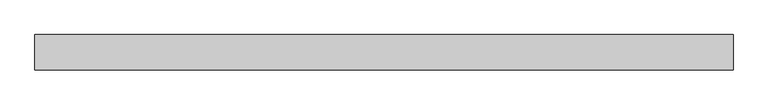
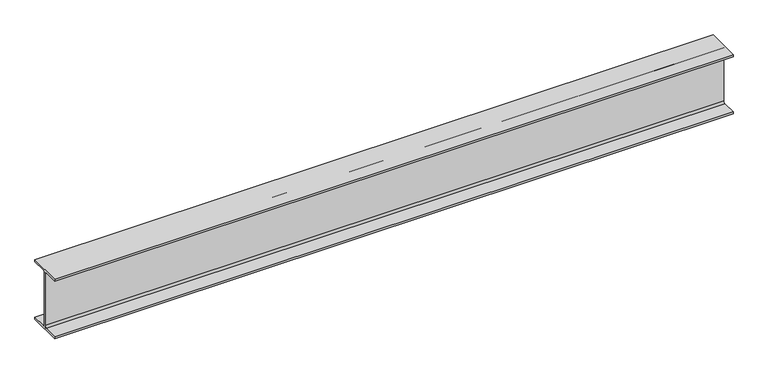
"""IFC4 building model written with IfcOpenShell, lengths in millimetres: beam geometry, Steel Beam_H-KSD3502 : H_SB_ASB_H-200x200x8x12."""

import ifcopenshell
import ifcopenshell.guid

model = None  # the IFC model being written
_history = None  # IfcOwnerHistory: only IFC2X3 demands one
_inside = {}  # id of a spatial element -> (the spatial element, [elements in it])
_under = {}  # id of a project, library or spatial element -> (it, [spatial elements below it])
_declared = {}  # id of a project -> (the project, [libraries it declares])
_typed = {}  # id of a type object -> (the type object, [elements of that type])
_made_of = {}  # id of a material, layer set ... -> (it, [elements and type objects made of it])


def new_model(schema):
    """Start an empty IFC model of exactly this schema.

    Asked for "IFC4X3", IfcOpenShell would pick the latest addendum, in which some entities
    have other attributes; the version numbers below select the first issue.
    IFC2X3 requires an IfcOwnerHistory on every rooted entity: one is made here for all.
    """
    global model, _history
    if schema == "IFC4X3":
        model = ifcopenshell.file(schema_version=(4, 3, 0, 0))
    else:
        model = ifcopenshell.file(schema=schema)
    _inside.clear()
    _under.clear()
    _declared.clear()
    _typed.clear()
    _made_of.clear()
    _history = None
    if model.schema == "IFC2X3":
        org = make("IfcOrganization", Name="unknown")
        user = make(
            "IfcPersonAndOrganization",
            ThePerson=make("IfcPerson", FamilyName="unknown"),
            TheOrganization=org,
        )
        app = make(
            "IfcApplication",
            ApplicationDeveloper=org,
            Version="unknown",
            ApplicationFullName="unknown",
            ApplicationIdentifier="unknown",
        )
        _history = make(
            "IfcOwnerHistory",
            OwningUser=user,
            OwningApplication=app,
            ChangeAction="ADDED",
            CreationDate=0,
        )
    return model


def make(cls, **values):
    """One entity of the class cls with the attributes given. An attribute that is None is left unset."""
    return model.create_entity(
        cls, **{name: value for name, value in values.items() if value is not None}
    )


def rooted(cls, **values):
    """An entity with a GlobalId (a new one), such as an element, a storey or a relation."""
    return make(cls, GlobalId=ifcopenshell.guid.new(), OwnerHistory=_history, **values)


def si_unit(unit_type, name, prefix=None):
    """IfcSIUnit, for example si_unit("LENGTHUNIT", "METRE", prefix="MILLI")."""
    return make("IfcSIUnit", UnitType=unit_type, Prefix=prefix, Name=name)


def assignment(units):
    """IfcUnitAssignment: the units of a project."""
    return None if units is None else make("IfcUnitAssignment", Units=units)


def point(xyz):
    """IfcCartesianPoint."""
    return None if xyz is None else make("IfcCartesianPoint", Coordinates=xyz)


def direction(xyz):
    """IfcDirection."""
    return None if xyz is None else make("IfcDirection", DirectionRatios=xyz)


def frame(location, z_axis=None, x_axis=None):
    """IfcAxis2Placement3D, a coordinate frame: its origin and axes. An axis left out is left unset."""
    return make(
        "IfcAxis2Placement3D",
        Location=point(location),
        Axis=direction(z_axis),
        RefDirection=direction(x_axis),
    )


def frame_2d(location, x_axis=None):
    """IfcAxis2Placement2D, a coordinate frame in the plane: its origin and x axis."""
    return make(
        "IfcAxis2Placement2D", Location=point(location), RefDirection=direction(x_axis)
    )


def origin():
    """The frame at (0, 0, 0) with its axes left unset."""
    return frame((0.0, 0.0, 0.0))


def place(relative_to, where):
    """IfcLocalPlacement: puts the frame where relative to a parent placement (None: the world)."""
    return make(
        "IfcLocalPlacement", PlacementRelTo=relative_to, RelativePlacement=where
    )


def context(
    kind, dimensions, precision=None, world=None, true_north=None, identifier=None
):
    """IfcGeometricRepresentationContext, for example the 3D "Model" context."""
    return make(
        "IfcGeometricRepresentationContext",
        ContextIdentifier=identifier,
        ContextType=kind,
        CoordinateSpaceDimension=dimensions,
        Precision=precision,
        WorldCoordinateSystem=world,
        TrueNorth=true_north,
    )


def project(units=None, contexts=None):
    """IfcProject with its units and contexts."""
    return rooted(
        "IfcProject",
        Name="project",
        RepresentationContexts=contexts,
        UnitsInContext=assignment(units),
    )


def spatial(cls, under=None, at=None, **own):
    """A site, building, storey or space (cls), placed at a placement, below another one or the project."""
    s = rooted(cls, ObjectPlacement=at, **own)
    if under is not None:
        _under.setdefault(under.id(), (under, []))[1].append(s)
    return s


def polyline(points):
    """IfcPolyline through the points."""
    return make("IfcPolyline", Points=[point(p) for p in points])


def circle_curve(where, radius):
    """IfcCircle in the frame where."""
    return make("IfcCircle", Position=where, Radius=radius)


def trimmed(basis, trim1, trim2, sense, master):
    """IfcTrimmedCurve: the piece of a basis curve between two trims."""
    return make(
        "IfcTrimmedCurve",
        BasisCurve=basis,
        Trim1=trim1,
        Trim2=trim2,
        SenseAgreement=sense,
        MasterRepresentation=master,
    )


def segment(curve, same_sense, transition):
    """IfcCompositeCurveSegment."""
    return make(
        "IfcCompositeCurveSegment",
        Transition=transition,
        SameSense=same_sense,
        ParentCurve=curve,
    )


def composite_curve(segments, self_intersect=None):
    """IfcCompositeCurve: segments joined end to end."""
    return make("IfcCompositeCurve", Segments=segments, SelfIntersect=self_intersect)


def outline(outer, holes=None, kind="AREA"):
    """IfcArbitraryClosedProfileDef: a profile drawn as a closed curve; with holes, ...WithVoids."""
    if holes is None:
        return make("IfcArbitraryClosedProfileDef", ProfileType=kind, OuterCurve=outer)
    return make(
        "IfcArbitraryProfileDefWithVoids",
        ProfileType=kind,
        OuterCurve=outer,
        InnerCurves=holes,
    )


def extrude(swept, where, along, depth):
    """IfcExtrudedAreaSolid: the profile swept, set in the frame where, extruded along a direction by depth."""
    return make(
        "IfcExtrudedAreaSolid",
        SweptArea=swept,
        Position=where,
        ExtrudedDirection=direction(along),
        Depth=depth,
    )


def shape(context_of_items, identifier, shape_type, items):
    """IfcShapeRepresentation: the items that make up one representation, for example the "Body"."""
    return make(
        "IfcShapeRepresentation",
        ContextOfItems=context_of_items,
        RepresentationIdentifier=identifier,
        RepresentationType=shape_type,
        Items=items,
    )


def source(mapping_origin, context_of_items, identifier, shape_type, items):
    """IfcRepresentationMap: a shape defined once, which mapped items show again and again."""
    return make(
        "IfcRepresentationMap",
        MappingOrigin=mapping_origin,
        MappedRepresentation=shape(context_of_items, identifier, shape_type, items),
    )


def transform(
    local_origin,
    x_axis=None,
    y_axis=None,
    z_axis=None,
    scale=None,
    scale2=None,
    scale3=None,
    uniform=True,
):
    """IfcCartesianTransformationOperator3D, or its non-uniform kind. x_axis, y_axis, z_axis: its Axis1, 2, 3."""
    if uniform:
        return make(
            "IfcCartesianTransformationOperator3D",
            Axis1=direction(x_axis),
            Axis2=direction(y_axis),
            LocalOrigin=point(local_origin),
            Scale=scale,
            Axis3=direction(z_axis),
        )
    return make(
        "IfcCartesianTransformationOperator3DnonUniform",
        Axis1=direction(x_axis),
        Axis2=direction(y_axis),
        LocalOrigin=point(local_origin),
        Scale=scale,
        Axis3=direction(z_axis),
        Scale2=scale2,
        Scale3=scale3,
    )


def mapped(mapping_source, mapping_target):
    """IfcMappedItem: shows the shape of a source again, moved by a transform."""
    return make(
        "IfcMappedItem", MappingSource=mapping_source, MappingTarget=mapping_target
    )


def made_of(thing, what):
    """Note that an element or type object is made of a material, layer set ...; save() writes the relation."""
    if what is not None:
        _made_of.setdefault(what.id(), (what, []))[1].append(thing)
    return thing


def element(
    cls,
    number,
    at=None,
    inside=None,
    cuts=None,
    type_object=None,
    material=None,
    context=None,
    identifier="Body",
    shape_type=None,
    held_by="IfcProductDefinitionShape",
    body=None,
    shapes=None,
    **own,
):
    """One element of the class cls, such as IfcWall. Its Tag is "e" and its number.

    at: its placement. inside: the storey or other place that contains it. cuts: it is an
    opening in that element (IfcRelVoidsElement). A single representation is given by context,
    identifier, shape_type and body (its items); several are given by shapes. held_by: the class
    of the entity that holds the representations. save() writes the other relations.
    """
    e = rooted(cls, Tag="e%d" % number, ObjectPlacement=at, **own)
    if body is not None:
        shapes = [shape(context, identifier, shape_type, body)]
    if shapes is not None:
        e.Representation = make(held_by, Representations=shapes)
    if inside is not None:
        _inside.setdefault(inside.id(), (inside, []))[1].append(e)
    if cuts is not None:
        rooted(
            "IfcRelVoidsElement", RelatingBuildingElement=cuts, RelatedOpeningElement=e
        )
    if type_object is not None:
        _typed.setdefault(type_object.id(), (type_object, []))[1].append(e)
    return made_of(e, material)


def aggregate(whole, parts):
    """IfcRelAggregates: a whole, such as a stair, and the parts it consists of."""
    return rooted("IfcRelAggregates", RelatingObject=whole, RelatedObjects=parts)


def save(model, path):
    """Write the relations noted so far, then the file.

    IfcRelAggregates (storeys below a building ...), IfcRelContainedInSpatialStructure (elements
    in a storey), IfcRelDefinesByType, IfcRelAssociatesMaterial and IfcRelDeclares: one each for
    every whole, place, type object, material and project.
    """
    for whole, parts in _under.values():
        aggregate(whole, parts)
    for where, things in _inside.values():
        rooted(
            "IfcRelContainedInSpatialStructure",
            RelatedElements=things,
            RelatingStructure=where,
        )
    for kind, things in _typed.values():
        rooted("IfcRelDefinesByType", RelatedObjects=things, RelatingType=kind)
    for what, things in _made_of.values():
        rooted("IfcRelAssociatesMaterial", RelatedObjects=things, RelatingMaterial=what)
    for by, libraries in _declared.values():
        rooted("IfcRelDeclares", RelatingContext=by, RelatedDefinitions=libraries)
    model.write(path)


def beam_5fd4a863(model_context):
    return source(origin(), model_context, "Body", "SweptSolid", [
        extrude(outline(composite_curve([segment(polyline([(82.5, -141.5), (82.5, -151.7), (-82.5, -151.7), (-82.5, -141.5), (-11.9, -141.5)]), True, "CONTINUOUS"), segment(trimmed(circle_curve(frame_2d((-11.9, -132.6)), 8.9), [point((-11.9, -141.5))], [point((-3.0, -132.6))], True, "CARTESIAN"), True, "CONTINUOUS"), segment(polyline([(-3.0, -132.6), (-3.0, 132.6)]), True, "CONTINUOUS"), segment(trimmed(circle_curve(frame_2d((-11.9, 132.6)), 8.9), [point((-3.0, 132.6))], [point((-11.9, 141.5))], True, "CARTESIAN"), True, "CONTINUOUS"), segment(polyline([(-11.9, 141.5), (-82.5, 141.5), (-82.5, 151.7), (82.5, 151.7), (82.5, 141.5), (11.9, 141.5)]), True, "CONTINUOUS"), segment(trimmed(circle_curve(frame_2d((11.9, 132.6)), 8.9), [point((11.9, 141.5))], [point((3.0, 132.6))], True, "CARTESIAN"), True, "CONTINUOUS"), segment(polyline([(3.0, 132.6), (3.0, -132.6)]), True, "CONTINUOUS"), segment(trimmed(circle_curve(frame_2d((11.9, -132.6)), 8.9), [point((3.0, -132.6))], [point((11.9, -141.5))], True, "CARTESIAN"), True, "CONTINUOUS"), segment(polyline([(11.9, -141.5), (82.5, -141.5)]), True, "CONTINUOUS")], self_intersect=False)), frame((-1689.2318964, 0.0, 0.0), z_axis=(1.0, 0.0, 0.0), x_axis=(0.0, 1.0, 0.0)), (0.0, 0.0, 1.0), 3273.7082384),
    ])


if __name__ == "__main__":
    model = new_model("IFC4")
    model_context = context("Model", 3, world=origin())
    ifc_project = project(units=[si_unit("LENGTHUNIT", "METRE", prefix="MILLI")], contexts=[model_context])
    site = spatial("IfcSite", under=ifc_project)
    building = spatial("IfcBuilding", under=site)
    placement = place(None, origin())
    beam_shape = beam_5fd4a863(model_context)
    element("IfcBeam", 1, ObjectType="Steel Beam_H-KSD3502 : H_SB_ASB_H-200x200x8x12", at=placement, inside=building, context=model_context, shape_type="MappedRepresentation", body=[
        mapped(beam_shape, transform((0.0, 0.0, 0.0), x_axis=(1.0, 0.0, 0.0), y_axis=(0.0, 1.0, 0.0), z_axis=(0.0, 0.0, 1.0))),
    ])
    save(model, "model.ifc")

# Revit data of these elements
# Type "Steel Beam_H-KSD3502 : H_SB_ASB_H-200x200x8x12"
#   Width = 20.0 cm
#   Web Thickness = 0.8 cm
#   Web Fillet = 1.3 cm
#   Warping Constant = 141376.0 cm⁶
#   Torsional Moment of Inertia = 26.2485 cm⁴
#   Torsional Modulus = 1.0 cm³
#   Section Area = 63.53 cm²
#   Plastic Modulus weak axis = 244.0 cm³
#   Plastic Modulus strong axis = 525.0 cm³
#   Perimeter = 1.16 m²/m
#   Nominal Weight = 49.90 kgf/m
#   Moment of Inertia weak axis = 1600.00 cm⁴
#   Moment of Inertia strong axis = 4720.00 cm⁴
#   Height = 20.0 cm
#   Flange Thickness = 1.2 cm
#   Elastic Modulus weak axis = 160.0 cm³
#   Elastic Modulus strong axis = 472.0 cm³
#   Centroid Vertical = 10.0 cm
#   Centroid Horizontal = 10.0 cm
#   Length [instance default] = 1.5240 m
#   Structural Material [instance default] = Steel, 45-345
#   Assembly Code = ""
# Element 1 (IfcBeam, "Steel Beam_H-KSD3502 : H_SB_ASB_H-200x200x8x12")
#   Structural Material = none
# Materials
#   "Steel, 45-345": class "Metal", colour RGB 189 187 185, transparency 0, Description = "Steel 345 MPa", Cost = 0
